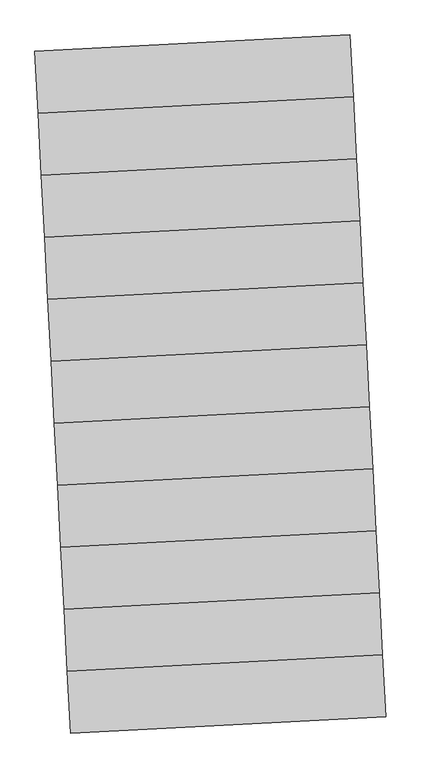
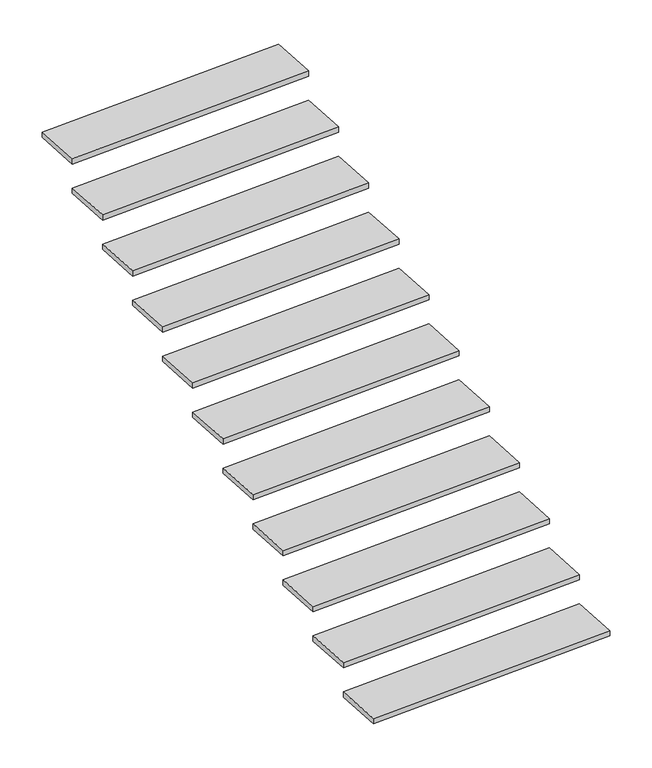
"""IFC4 building model written with IfcOpenShell, lengths in millimetres: stair flight geometry."""

from ifc_helpers import new_model, si_unit, frame, origin, place, context, project, spatial, polyline, outline, extrude, source, transform, mapped, element, save


def stair_flight_18440aeb(model_context):
    return source(origin(), model_context, "Body", "SweptSolid", [
        extrude(outline(polyline([(21524.3114867, 12733.1881413), (22897.427097, 12805.1500812), (22911.5578051, 12535.5201068), (21538.4421949, 12463.5581669), (21524.3114867, 12733.1881413)])), frame((0.0, 0.0, -157.0), z_axis=(0.0, 0.0, 1.0), x_axis=(1.0, 0.0, 0.0)), (0.0, 0.0, 1.0), 32.0),
        extrude(outline(polyline([(21510.1807785, 13002.8181157), (22883.2963888, 13074.7800555), (22897.427097, 12805.1500812), (21524.3114867, 12733.1881413), (21510.1807785, 13002.8181157)])), frame((0.0, 0.0, 18.0), z_axis=(0.0, 0.0, 1.0), x_axis=(1.0, 0.0, 0.0)), (0.0, 0.0, 1.0), 32.0),
        extrude(outline(polyline([(21496.0500703, 13272.4480901), (22869.1656806, 13344.4100299), (22883.2963888, 13074.7800555), (21510.1807785, 13002.8181157), (21496.0500703, 13272.4480901)])), frame((0.0, 0.0, 193.0), z_axis=(0.0, 0.0, 1.0), x_axis=(1.0, 0.0, 0.0)), (0.0, 0.0, 1.0), 32.0),
        extrude(outline(polyline([(21481.9193621, 13542.0780645), (22855.0349724, 13614.0400043), (22869.1656806, 13344.4100299), (21496.0500703, 13272.4480901), (21481.9193621, 13542.0780645)])), frame((0.0, 0.0, 368.0), z_axis=(0.0, 0.0, 1.0), x_axis=(1.0, 0.0, 0.0)), (0.0, 0.0, 1.0), 32.0),
        extrude(outline(polyline([(21467.7886539, 13811.7080389), (22840.9042642, 13883.6699787), (22855.0349724, 13614.0400043), (21481.9193621, 13542.0780645), (21467.7886539, 13811.7080389)])), frame((0.0, 0.0, 543.0), z_axis=(0.0, 0.0, 1.0), x_axis=(1.0, 0.0, 0.0)), (0.0, 0.0, 1.0), 32.0),
        extrude(outline(polyline([(21453.6579457, 14081.3380132), (22826.773556, 14153.2999531), (22840.9042642, 13883.6699787), (21467.7886539, 13811.7080389), (21453.6579457, 14081.3380132)])), frame((0.0, 0.0, 718.0), z_axis=(0.0, 0.0, 1.0), x_axis=(1.0, 0.0, 0.0)), (0.0, 0.0, 1.0), 32.0),
        extrude(outline(polyline([(21439.5272376, 14350.9679876), (22812.6428478, 14422.9299275), (22826.773556, 14153.2999531), (21453.6579457, 14081.3380132), (21439.5272376, 14350.9679876)])), frame((0.0, 0.0, 893.0), z_axis=(0.0, 0.0, 1.0), x_axis=(1.0, 0.0, 0.0)), (0.0, 0.0, 1.0), 32.0),
        extrude(outline(polyline([(21425.3965294, 14620.597962), (22798.5121397, 14692.5599018), (22812.6428478, 14422.9299275), (21439.5272376, 14350.9679876), (21425.3965294, 14620.597962)])), frame((0.0, 0.0, 1068.0), z_axis=(0.0, 0.0, 1.0), x_axis=(1.0, 0.0, 0.0)), (0.0, 0.0, 1.0), 32.0),
        extrude(outline(polyline([(21411.2658212, 14890.2279364), (22784.3814315, 14962.1898762), (22798.5121397, 14692.5599018), (21425.3965294, 14620.597962), (21411.2658212, 14890.2279364)])), frame((0.0, 0.0, 1243.0), z_axis=(0.0, 0.0, 1.0), x_axis=(1.0, 0.0, 0.0)), (0.0, 0.0, 1.0), 32.0),
        extrude(outline(polyline([(21397.135113, 15159.8579108), (22770.2507233, 15231.8198506), (22784.3814315, 14962.1898762), (21411.2658212, 14890.2279364), (21397.135113, 15159.8579108)])), frame((0.0, 0.0, 1418.0), z_axis=(0.0, 0.0, 1.0), x_axis=(1.0, 0.0, 0.0)), (0.0, 0.0, 1.0), 32.0),
        extrude(outline(polyline([(21383.0044048, 15429.4878852), (22756.1200151, 15501.449825), (22770.2507233, 15231.8198506), (21397.135113, 15159.8579108), (21383.0044048, 15429.4878852)])), frame((0.0, 0.0, 1593.0), z_axis=(0.0, 0.0, 1.0), x_axis=(1.0, 0.0, 0.0)), (0.0, 0.0, 1.0), 32.0),
    ])


if __name__ == "__main__":
    model = new_model("IFC4")
    model_context = context("Model", 3, world=origin())
    ifc_project = project(units=[si_unit("LENGTHUNIT", "METRE", prefix="MILLI")], contexts=[model_context])
    site = spatial("IfcSite", under=ifc_project)
    building = spatial("IfcBuilding", under=site)
    placement = place(None, origin())
    stair_flight_shape = stair_flight_18440aeb(model_context)
    element("IfcStairFlight", 1, at=placement, inside=building, context=model_context, shape_type="MappedRepresentation", body=[
        mapped(stair_flight_shape, transform((0.0, 0.0, 0.0), x_axis=(1.0, 0.0, 0.0), y_axis=(0.0, 1.0, 0.0), z_axis=(0.0, 0.0, 1.0))),
    ])
    save(model, "model.ifc")

# Revit data of these elements
# Element 1 (IfcStairFlight)
#   Materials on its faces: "철강"
# Materials
#   "철강": class "Generic", colour RGB 143 142 141, transparency 0, Description = "철골+가공조립+세우기", Cost = 0
